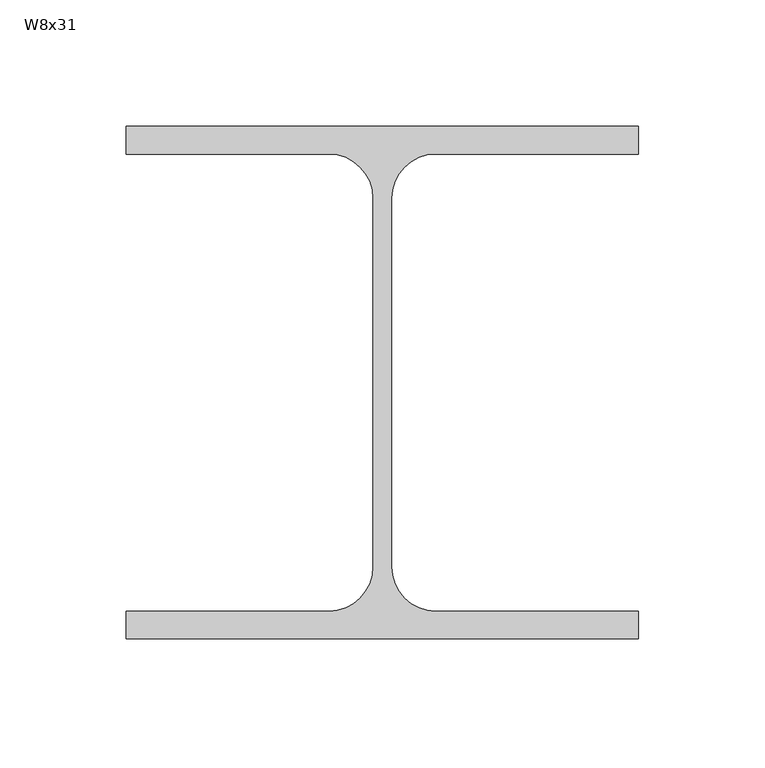
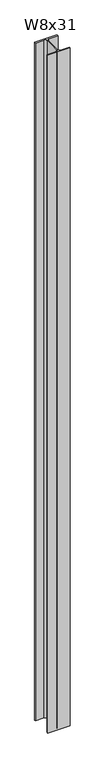
"""IFC4 building model written with IfcOpenShell, lengths in millimetres: column geometry, RME WF - Column : W8x31."""

import ifcopenshell
import ifcopenshell.guid

model = None  # the IFC model being written
_history = None  # IfcOwnerHistory: only IFC2X3 demands one
_inside = {}  # id of a spatial element -> (the spatial element, [elements in it])
_under = {}  # id of a project, library or spatial element -> (it, [spatial elements below it])
_declared = {}  # id of a project -> (the project, [libraries it declares])
_typed = {}  # id of a type object -> (the type object, [elements of that type])
_made_of = {}  # id of a material, layer set ... -> (it, [elements and type objects made of it])


def new_model(schema):
    """Start an empty IFC model of exactly this schema.

    Asked for "IFC4X3", IfcOpenShell would pick the latest addendum, in which some entities
    have other attributes; the version numbers below select the first issue.
    IFC2X3 requires an IfcOwnerHistory on every rooted entity: one is made here for all.
    """
    global model, _history
    if schema == "IFC4X3":
        model = ifcopenshell.file(schema_version=(4, 3, 0, 0))
    else:
        model = ifcopenshell.file(schema=schema)
    _inside.clear()
    _under.clear()
    _declared.clear()
    _typed.clear()
    _made_of.clear()
    _history = None
    if model.schema == "IFC2X3":
        org = make("IfcOrganization", Name="unknown")
        user = make(
            "IfcPersonAndOrganization",
            ThePerson=make("IfcPerson", FamilyName="unknown"),
            TheOrganization=org,
        )
        app = make(
            "IfcApplication",
            ApplicationDeveloper=org,
            Version="unknown",
            ApplicationFullName="unknown",
            ApplicationIdentifier="unknown",
        )
        _history = make(
            "IfcOwnerHistory",
            OwningUser=user,
            OwningApplication=app,
            ChangeAction="ADDED",
            CreationDate=0,
        )
    return model


def make(cls, **values):
    """One entity of the class cls with the attributes given. An attribute that is None is left unset."""
    return model.create_entity(
        cls, **{name: value for name, value in values.items() if value is not None}
    )


def rooted(cls, **values):
    """An entity with a GlobalId (a new one), such as an element, a storey or a relation."""
    return make(cls, GlobalId=ifcopenshell.guid.new(), OwnerHistory=_history, **values)


def si_unit(unit_type, name, prefix=None):
    """IfcSIUnit, for example si_unit("LENGTHUNIT", "METRE", prefix="MILLI")."""
    return make("IfcSIUnit", UnitType=unit_type, Prefix=prefix, Name=name)


def assignment(units):
    """IfcUnitAssignment: the units of a project."""
    return None if units is None else make("IfcUnitAssignment", Units=units)


def point(xyz):
    """IfcCartesianPoint."""
    return None if xyz is None else make("IfcCartesianPoint", Coordinates=xyz)


def direction(xyz):
    """IfcDirection."""
    return None if xyz is None else make("IfcDirection", DirectionRatios=xyz)


def frame(location, z_axis=None, x_axis=None):
    """IfcAxis2Placement3D, a coordinate frame: its origin and axes. An axis left out is left unset."""
    return make(
        "IfcAxis2Placement3D",
        Location=point(location),
        Axis=direction(z_axis),
        RefDirection=direction(x_axis),
    )


def frame_2d(location, x_axis=None):
    """IfcAxis2Placement2D, a coordinate frame in the plane: its origin and x axis."""
    return make(
        "IfcAxis2Placement2D", Location=point(location), RefDirection=direction(x_axis)
    )


def origin():
    """The frame at (0, 0, 0) with its axes left unset."""
    return frame((0.0, 0.0, 0.0))


def place(relative_to, where):
    """IfcLocalPlacement: puts the frame where relative to a parent placement (None: the world)."""
    return make(
        "IfcLocalPlacement", PlacementRelTo=relative_to, RelativePlacement=where
    )


def context(
    kind, dimensions, precision=None, world=None, true_north=None, identifier=None
):
    """IfcGeometricRepresentationContext, for example the 3D "Model" context."""
    return make(
        "IfcGeometricRepresentationContext",
        ContextIdentifier=identifier,
        ContextType=kind,
        CoordinateSpaceDimension=dimensions,
        Precision=precision,
        WorldCoordinateSystem=world,
        TrueNorth=true_north,
    )


def project(units=None, contexts=None):
    """IfcProject with its units and contexts."""
    return rooted(
        "IfcProject",
        Name="project",
        RepresentationContexts=contexts,
        UnitsInContext=assignment(units),
    )


def spatial(cls, under=None, at=None, **own):
    """A site, building, storey or space (cls), placed at a placement, below another one or the project."""
    s = rooted(cls, ObjectPlacement=at, **own)
    if under is not None:
        _under.setdefault(under.id(), (under, []))[1].append(s)
    return s


def polyline(points):
    """IfcPolyline through the points."""
    return make("IfcPolyline", Points=[point(p) for p in points])


def circle_curve(where, radius):
    """IfcCircle in the frame where."""
    return make("IfcCircle", Position=where, Radius=radius)


def trimmed(basis, trim1, trim2, sense, master):
    """IfcTrimmedCurve: the piece of a basis curve between two trims."""
    return make(
        "IfcTrimmedCurve",
        BasisCurve=basis,
        Trim1=trim1,
        Trim2=trim2,
        SenseAgreement=sense,
        MasterRepresentation=master,
    )


def segment(curve, same_sense, transition):
    """IfcCompositeCurveSegment."""
    return make(
        "IfcCompositeCurveSegment",
        Transition=transition,
        SameSense=same_sense,
        ParentCurve=curve,
    )


def composite_curve(segments, self_intersect=None):
    """IfcCompositeCurve: segments joined end to end."""
    return make("IfcCompositeCurve", Segments=segments, SelfIntersect=self_intersect)


def outline(outer, holes=None, kind="AREA"):
    """IfcArbitraryClosedProfileDef: a profile drawn as a closed curve; with holes, ...WithVoids."""
    if holes is None:
        return make("IfcArbitraryClosedProfileDef", ProfileType=kind, OuterCurve=outer)
    return make(
        "IfcArbitraryProfileDefWithVoids",
        ProfileType=kind,
        OuterCurve=outer,
        InnerCurves=holes,
    )


def extrude(swept, where, along, depth):
    """IfcExtrudedAreaSolid: the profile swept, set in the frame where, extruded along a direction by depth."""
    return make(
        "IfcExtrudedAreaSolid",
        SweptArea=swept,
        Position=where,
        ExtrudedDirection=direction(along),
        Depth=depth,
    )


def shape(context_of_items, identifier, shape_type, items):
    """IfcShapeRepresentation: the items that make up one representation, for example the "Body"."""
    return make(
        "IfcShapeRepresentation",
        ContextOfItems=context_of_items,
        RepresentationIdentifier=identifier,
        RepresentationType=shape_type,
        Items=items,
    )


def source(mapping_origin, context_of_items, identifier, shape_type, items):
    """IfcRepresentationMap: a shape defined once, which mapped items show again and again."""
    return make(
        "IfcRepresentationMap",
        MappingOrigin=mapping_origin,
        MappedRepresentation=shape(context_of_items, identifier, shape_type, items),
    )


def transform(
    local_origin,
    x_axis=None,
    y_axis=None,
    z_axis=None,
    scale=None,
    scale2=None,
    scale3=None,
    uniform=True,
):
    """IfcCartesianTransformationOperator3D, or its non-uniform kind. x_axis, y_axis, z_axis: its Axis1, 2, 3."""
    if uniform:
        return make(
            "IfcCartesianTransformationOperator3D",
            Axis1=direction(x_axis),
            Axis2=direction(y_axis),
            LocalOrigin=point(local_origin),
            Scale=scale,
            Axis3=direction(z_axis),
        )
    return make(
        "IfcCartesianTransformationOperator3DnonUniform",
        Axis1=direction(x_axis),
        Axis2=direction(y_axis),
        LocalOrigin=point(local_origin),
        Scale=scale,
        Axis3=direction(z_axis),
        Scale2=scale2,
        Scale3=scale3,
    )


def mapped(mapping_source, mapping_target):
    """IfcMappedItem: shows the shape of a source again, moved by a transform."""
    return make(
        "IfcMappedItem", MappingSource=mapping_source, MappingTarget=mapping_target
    )


def made_of(thing, what):
    """Note that an element or type object is made of a material, layer set ...; save() writes the relation."""
    if what is not None:
        _made_of.setdefault(what.id(), (what, []))[1].append(thing)
    return thing


def element(
    cls,
    number,
    at=None,
    inside=None,
    cuts=None,
    type_object=None,
    material=None,
    context=None,
    identifier="Body",
    shape_type=None,
    held_by="IfcProductDefinitionShape",
    body=None,
    shapes=None,
    **own,
):
    """One element of the class cls, such as IfcWall. Its Tag is "e" and its number.

    at: its placement. inside: the storey or other place that contains it. cuts: it is an
    opening in that element (IfcRelVoidsElement). A single representation is given by context,
    identifier, shape_type and body (its items); several are given by shapes. held_by: the class
    of the entity that holds the representations. save() writes the other relations.
    """
    e = rooted(cls, Tag="e%d" % number, ObjectPlacement=at, **own)
    if body is not None:
        shapes = [shape(context, identifier, shape_type, body)]
    if shapes is not None:
        e.Representation = make(held_by, Representations=shapes)
    if inside is not None:
        _inside.setdefault(inside.id(), (inside, []))[1].append(e)
    if cuts is not None:
        rooted(
            "IfcRelVoidsElement", RelatingBuildingElement=cuts, RelatedOpeningElement=e
        )
    if type_object is not None:
        _typed.setdefault(type_object.id(), (type_object, []))[1].append(e)
    return made_of(e, material)


def aggregate(whole, parts):
    """IfcRelAggregates: a whole, such as a stair, and the parts it consists of."""
    return rooted("IfcRelAggregates", RelatingObject=whole, RelatedObjects=parts)


def save(model, path):
    """Write the relations noted so far, then the file.

    IfcRelAggregates (storeys below a building ...), IfcRelContainedInSpatialStructure (elements
    in a storey), IfcRelDefinesByType, IfcRelAssociatesMaterial and IfcRelDeclares: one each for
    every whole, place, type object, material and project.
    """
    for whole, parts in _under.values():
        aggregate(whole, parts)
    for where, things in _inside.values():
        rooted(
            "IfcRelContainedInSpatialStructure",
            RelatedElements=things,
            RelatingStructure=where,
        )
    for kind, things in _typed.values():
        rooted("IfcRelDefinesByType", RelatedObjects=things, RelatingType=kind)
    for what, things in _made_of.values():
        rooted("IfcRelAssociatesMaterial", RelatedObjects=things, RelatingMaterial=what)
    for by, libraries in _declared.values():
        rooted("IfcRelDeclares", RelatingContext=by, RelatedDefinitions=libraries)
    model.write(path)


def w8x31_abfa5b44(model_context):
    return source(origin(), model_context, "Body", "SweptSolid", [
        extrude(outline(composite_curve([segment(polyline([(101.6, 101.6), (101.6, 90.551), (21.1455, 90.551)]), True, "CONTINUOUS"), segment(trimmed(circle_curve(frame_2d((21.1455, 73.025)), 17.526), [point((21.1455, 90.551))], [point((3.6195, 73.025))], True, "CARTESIAN"), True, "CONTINUOUS"), segment(polyline([(3.6195, 73.025), (3.6195, -73.025)]), True, "CONTINUOUS"), segment(trimmed(circle_curve(frame_2d((21.1455, -73.025)), 17.526), [point((3.6195, -73.025))], [point((21.1455, -90.551))], True, "CARTESIAN"), True, "CONTINUOUS"), segment(polyline([(21.1455, -90.551), (101.6, -90.551), (101.6, -101.6), (-101.6, -101.6), (-101.6, -90.551), (-21.1455, -90.551)]), True, "CONTINUOUS"), segment(trimmed(circle_curve(frame_2d((-21.1455, -73.025)), 17.526), [point((-21.1455, -90.551))], [point((-3.6195, -73.025))], True, "CARTESIAN"), True, "CONTINUOUS"), segment(polyline([(-3.6195, -73.025), (-3.6195, 73.025)]), True, "CONTINUOUS"), segment(trimmed(circle_curve(frame_2d((-21.1455, 73.025)), 17.526), [point((-3.6195, 73.025))], [point((-21.1455, 90.551))], True, "CARTESIAN"), True, "CONTINUOUS"), segment(polyline([(-21.1455, 90.551), (-101.6, 90.551), (-101.6, 101.6), (101.6, 101.6)]), True, "CONTINUOUS")], self_intersect=False)), frame((0.0, 0.0, -304.8), z_axis=(0.0, 0.0, 1.0), x_axis=(1.0, 0.0, 0.0)), (0.0, 0.0, 1.0), 6489.7),
    ])


if __name__ == "__main__":
    model = new_model("IFC4")
    model_context = context("Model", 3, world=origin())
    ifc_project = project(units=[si_unit("LENGTHUNIT", "METRE", prefix="MILLI")], contexts=[model_context])
    site = spatial("IfcSite", under=ifc_project)
    building = spatial("IfcBuilding", under=site)
    placement = place(None, origin())
    w8x31_shape = w8x31_abfa5b44(model_context)
    element("IfcColumn", 1, ObjectType="RME WF - Column : W8x31", at=placement, inside=building, context=model_context, shape_type="MappedRepresentation", body=[
        mapped(w8x31_shape, transform((0.0, 0.0, 0.0), x_axis=(1.0, 0.0, 0.0), y_axis=(0.0, 1.0, 0.0), z_axis=(0.0, 0.0, 1.0))),
    ])
    save(model, "model.ifc")

# Revit data of these elements
# Type "RME WF - Column : W8x31"
#   REINF TYPE [instance default] = ""
#   Nominal Size = "W16"
#   COL REMARKS [instance default] = ""
#   BP [instance default] = ""
#   Assembly Code = "B10"
#   W = 31
#   bf = 0' - 8"
#   d = 0' - 8"
#   k = 0' - 1 1/8"
#   kr = 0' - 0.69"
#   tf = 0' - 0.435"
#   tw = 0' - 0.285"
#   A = 0.0633333 SF
#   Structural Material [instance default] = Metal - Steel - ASTM A992
# Element 1 (IfcColumn, "RME WF - Column : W8x31")
#   Materials on its faces: "Metal - Steel - ASTM A992"
# Materials
#   "Metal - Steel - ASTM A992": class "Metal", colour RGB 255 128 0, transparency 0
